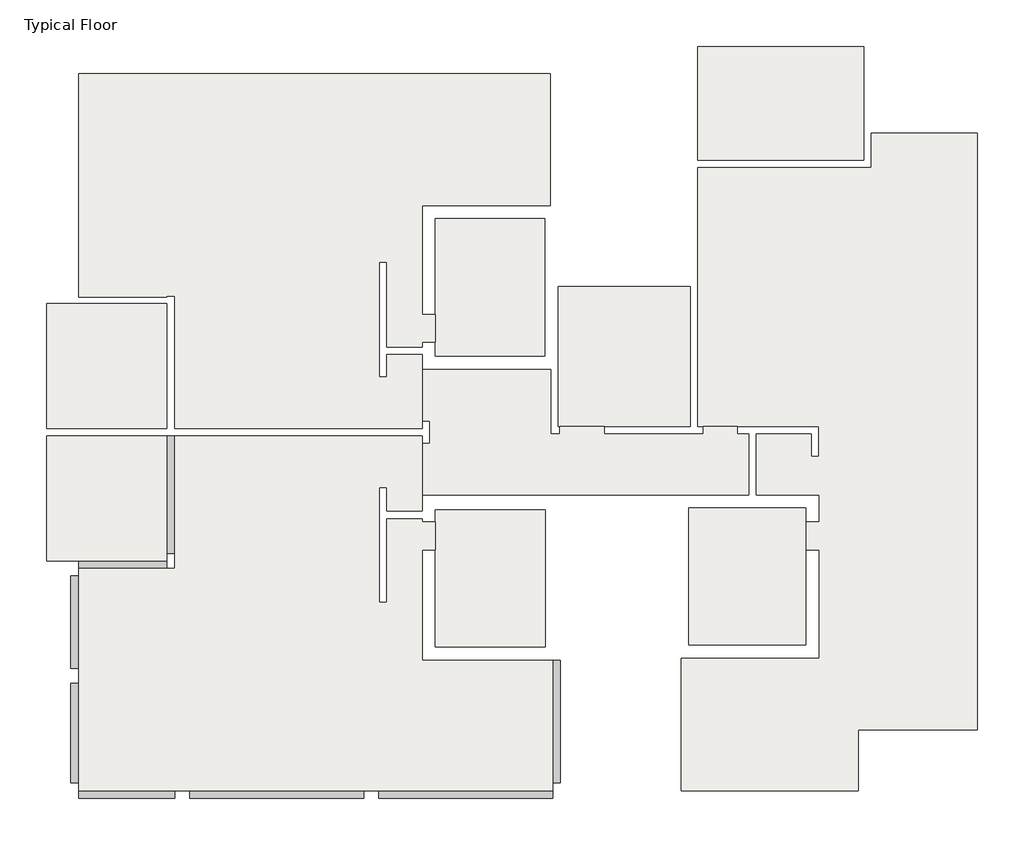
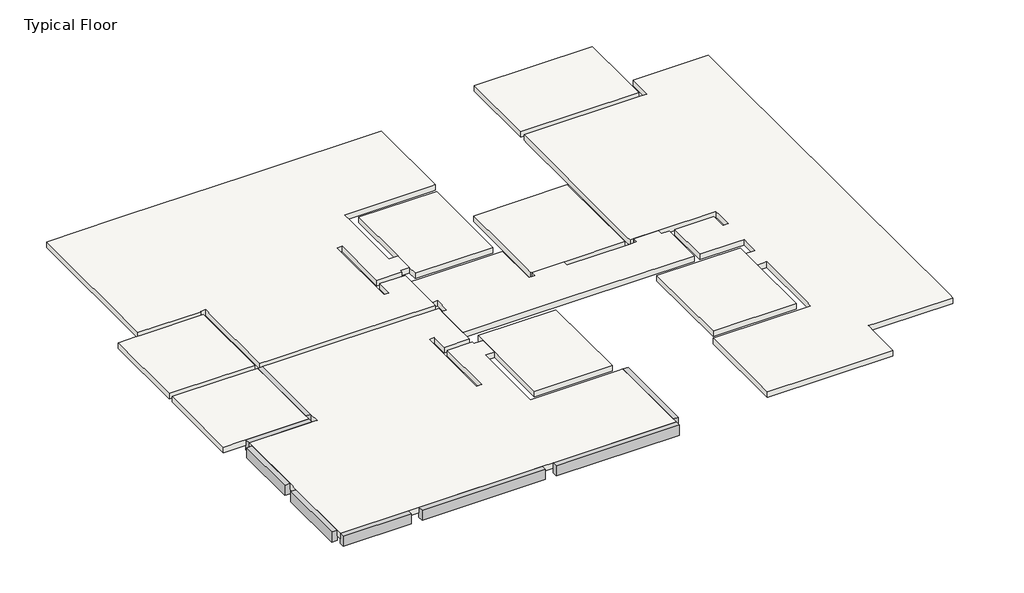
# One storey: 11 slabs, 8 beams.
"""IFC4 building model written with IfcOpenShell, lengths in millimetres."""

from ifc_helpers import new_model, si_unit, frame, origin, place, context, project, spatial, polyline, outline, extrude, faceted_brep, element, save

model = new_model("IFC4")

# Units and contexts
model_context = context("Model", 3, world=origin())
ifc_project = project(units=[si_unit("LENGTHUNIT", "METRE", prefix="MILLI")], contexts=[model_context])

# Site, building, storey
site = spatial("IfcSite", under=ifc_project)
building = spatial("IfcBuilding", under=site)
storey = spatial("IfcBuildingStorey", under=building, Name="Typical Floor", Elevation=3000.0)

# Beams
placement = place(None, origin())
element("IfcBeam", 1, ObjectType="Concrete Rectengular Beam : 20/40", at=placement, inside=storey, context=model_context, shape_type="SweptSolid", body=[
    extrude(outline(polyline([(-8952.4882749, -8486.1299304), (-8952.4882749, -8286.1299304), (-4346.8056177, -8286.1299304), (-4346.8056177, -8486.1299304), (-8952.4882749, -8486.1299304)])), frame((0.0, 0.0, 2600.0), z_axis=(0.0, 0.0, 1.0), x_axis=(1.0, 0.0, 0.0)), (0.0, 0.0, 1.0), 400.0),
])
element("IfcBeam", 2, ObjectType="Concrete Rectengular Beam : 20/40", at=placement, inside=storey, context=model_context, shape_type="Brep", body=[
    faceted_brep([(-11896.6244933, -8286.1299304, 3000.0), (-11896.6244933, -8486.1299304, 3000.0), (-9352.4882749, -8486.1299304, 3000.0), (-9352.4882749, -8286.1299304, 3000.0), (-11896.6244933, -8486.1299304, 2600.0), (-9352.4882749, -8486.1299304, 2600.0), (-11896.6244933, -8286.1299304, 2600.0), (-9352.4882749, -8286.1299304, 2600.0), (-11896.6244933, -8286.1299304, 2780.0)], [[[0, 1, 2, 3]], [[1, 4, 5, 2]], [[4, 6, 7, 5]], [[6, 8, 0, 3, 7]], [[1, 0, 8, 6, 4]], [[3, 2, 5, 7]]]),
])
element("IfcBeam", 3, ObjectType="Concrete Rectengular Beam : 20/40", at=placement, inside=storey, context=model_context, shape_type="SweptSolid", body=[
    extrude(outline(polyline([(-11896.6244933, -8086.1299304), (-12096.6244933, -8086.1299304), (-12096.6244933, -5448.6194614), (-11896.6244933, -5448.6194614), (-11896.6244933, -8086.1299304)])), frame((0.0, 0.0, 2600.0), z_axis=(0.0, 0.0, 1.0), x_axis=(1.0, 0.0, 0.0)), (0.0, 0.0, 1.0), 400.0),
])
element("IfcBeam", 4, ObjectType="Concrete Rectengular Beam : 20/40", at=placement, inside=storey, context=model_context, shape_type="SweptSolid", body=[
    extrude(outline(polyline([(-11896.6244933, -5048.6194614), (-12096.6244933, -5048.6194614), (-12096.6244933, -2598.4826712), (-11896.6244933, -2598.4826712), (-11896.6244933, -5048.6194614)])), frame((0.0, 0.0, 2600.0), z_axis=(0.0, 0.0, 1.0), x_axis=(1.0, 0.0, 0.0)), (0.0, 0.0, 1.0), 400.0),
])
element("IfcBeam", 5, ObjectType="Concrete Rectengular Beam : 20/40", at=placement, inside=storey, context=model_context, shape_type="Brep", body=[
    faceted_brep([(-9554.6843469, -2398.4826712, 3000.0), (-9554.6843469, -2198.4826712, 3000.0), (-11896.6244933, -2198.4826712, 3000.0), (-11896.6244933, -2398.4826712, 3000.0), (-9554.6843469, -2398.4826712, 2600.0), (-9554.6843469, -2398.4826712, 2780.0), (-11896.6244933, -2398.4826712, 2780.0), (-11896.6244933, -2398.4826712, 2600.0), (-9554.6843469, -2198.4826712, 2600.0), (-11896.6244933, -2198.4826712, 2600.0), (-9554.6843469, -2198.4826712, 2780.0)], [[[0, 1, 2, 3]], [[4, 5, 0, 3, 6, 7]], [[8, 4, 7, 9]], [[1, 10, 8, 9, 2]], [[1, 0, 5, 4, 8, 10]], [[3, 2, 9, 7, 6]]]),
])
element("IfcBeam", 6, ObjectType="Concrete Rectengular Beam : 20/40", at=placement, inside=storey, context=model_context, shape_type="Brep", body=[
    faceted_brep([(-9554.6843469, -1998.4826712, 3000.0), (-9354.6843469, -1998.4826712, 3000.0), (-9354.6843469, 1106.8737687, 3000.0), (-9554.6843469, 1106.8737687, 3000.0), (-9554.6843469, -1998.4826712, 2600.0), (-9554.6843469, 1106.8737687, 2780.0), (-9554.6843469, 1106.8737687, 2600.0), (-9354.6843469, -1998.4826712, 2600.0), (-9354.6843469, 1106.8737687, 2600.0), (-9354.6843469, -1998.4826712, 2780.0), (-9354.6843469, 1106.8737687, 2780.0)], [[[0, 1, 2, 3]], [[4, 0, 3, 5, 6]], [[7, 4, 6, 8]], [[1, 9, 7, 8, 10, 2]], [[1, 0, 4, 7, 9]], [[2, 10, 8, 6, 5, 3]]]),
])
element("IfcBeam", 7, ObjectType="Concrete Rectengular Beam : 20/40", at=placement, inside=storey, context=model_context, shape_type="Brep", body=[
    faceted_brep([(-3946.8056177, -8286.1299304, 3000.0), (-3946.8056177, -8486.1299304, 3000.0), (652.6741008, -8486.1299304, 3000.0), (652.6741008, -8286.1299304, 3000.0), (-3946.8056177, -8286.1299304, 2600.0), (652.6741008, -8286.1299304, 2780.0), (652.6741008, -8286.1299304, 2600.0), (-3946.8056177, -8486.1299304, 2600.0), (652.6741008, -8486.1299304, 2600.0)], [[[0, 1, 2, 3]], [[4, 0, 3, 5, 6]], [[7, 4, 6, 8]], [[1, 7, 8, 2]], [[1, 0, 4, 7]], [[3, 2, 8, 6, 5]]]),
])
element("IfcBeam", 8, ObjectType="Concrete Rectengular Beam : 20/40", at=placement, inside=storey, context=model_context, shape_type="Brep", body=[
    faceted_brep([(652.6741008, -8086.1299304, 3000.0), (852.6741008, -8086.1299304, 3000.0), (852.6741008, -4834.488398, 3000.0), (652.6741008, -4834.488398, 3000.0), (652.6741008, -8086.1299304, 2600.0), (652.6741008, -4834.488398, 2780.0), (652.6741008, -4834.488398, 2600.0), (852.6741008, -8086.1299304, 2600.0), (852.6741008, -4834.488398, 2600.0)], [[[0, 1, 2, 3]], [[4, 0, 3, 5, 6]], [[7, 4, 6, 8]], [[1, 7, 8, 2]], [[1, 0, 4, 7]], [[3, 2, 8, 6, 5]]]),
])

# Slabs
element("IfcSlab", 9, ObjectType="22", at=placement, inside=storey, context=model_context, shape_type="SweptSolid", body=[
    extrude(outline(polyline([(447.6741008, 6858.2359353), (447.6741008, 3218.2359353), (-2452.3258992, 3218.2359353), (-2452.3258992, 3588.2359353), (-2457.3258992, 3588.2359353), (-2457.3258992, 4328.2359353), (-2452.3258992, 4328.2359353), (-2452.3258992, 6858.2359353), (447.6741008, 6858.2359353)])), frame((0.0, 0.0, 2780.0), z_axis=(0.0, 0.0, 1.0), x_axis=(1.0, 0.0, 0.0)), (0.0, 0.0, 1.0), 220.0),
])
element("IfcSlab", 10, ObjectType="22", at=placement, inside=storey, context=model_context, shape_type="Brep", body=[
    faceted_brep([(-2802.3258992, 3588.2359353, 2780.0), (-2802.3258992, 3468.2359353, 2780.0), (-3737.2404282, 3468.2359353, 2780.0), (-3737.2404282, 5714.0630881, 2780.0), (-3737.2404282, 5714.3058677, 2780.0), (-3937.2404282, 5714.3058677, 2780.0), (-3937.2404282, 5714.0630881, 2780.0), (-3937.2404282, 2665.7744518, 2780.0), (-3737.2404282, 2665.7744518, 2780.0), (-3737.2404282, 3268.2359353, 2780.0), (-2802.3258992, 3268.2359353, 2780.0), (-2802.3258992, 2868.2359353, 2780.0), (-2800.2213409, 2868.2359353, 2780.0), (-2800.2213409, 1506.8737687, 2780.0), (-2800.2213409, 1306.8737687, 2780.0), (-9354.6843469, 1306.8737687, 2780.0), (-9354.6843469, 4812.2302086, 2780.0), (-9554.6843469, 4812.2302086, 2780.0), (-9554.6843469, 4790.1128337, 2780.0), (-11896.6244933, 4790.1128337, 2780.0), (-11896.6244933, 4812.2302086, 2780.0), (-11896.6244933, 10699.8774677, 2780.0), (592.5229388, 10699.8774677, 2780.0), (592.5229388, 7208.2359353, 2780.0), (447.6741008, 7208.2359353, 2780.0), (-2802.3258992, 7208.2359353, 2780.0), (-2802.3258992, 6858.2359353, 2780.0), (-2802.3258992, 4328.2359353, 2780.0), (-2457.3258992, 4328.2359353, 2780.0), (-2457.3258992, 3588.2359353, 2780.0), (-2802.3258992, 3468.2359353, 3000.0), (-2802.3258992, 3588.2359353, 3000.0), (-2457.3258992, 3588.2359353, 3000.0), (-2457.3258992, 4328.2359353, 3000.0), (-2802.3258992, 4328.2359353, 3000.0), (-2802.3258992, 6858.2359353, 3000.0), (-2802.3258992, 7208.2359353, 3000.0), (447.6741008, 7208.2359353, 3000.0), (592.5229388, 7208.2359353, 3000.0), (592.5229388, 10499.8774677, 3000.0), (592.5229388, 10699.8774677, 3000.0), (-3946.8056177, 10699.8774677, 3000.0), (-4346.8056177, 10699.8774677, 3000.0), (-8952.4882749, 10699.8774677, 3000.0), (-9352.4882749, 10699.8774677, 3000.0), (-11896.6244933, 10699.8774677, 3000.0), (-11896.6244933, 10499.8774677, 3000.0), (-11896.6244933, 7862.3669988, 3000.0), (-11896.6244933, 7462.3669988, 3000.0), (-11896.6244933, 5012.2302086, 3000.0), (-11896.6244933, 4790.1128337, 3000.0), (-9554.6843469, 4790.1128337, 3000.0), (-9554.6843469, 4812.2302086, 3000.0), (-9354.6843469, 4812.2302086, 3000.0), (-9354.6843469, 4412.2302086, 3000.0), (-9354.6843469, 1306.8737687, 3000.0), (-8954.6843469, 1306.8737687, 3000.0), (-6260.2213409, 1306.8737687, 3000.0), (-5860.2213409, 1306.8737687, 3000.0), (-2800.2213409, 1306.8737687, 3000.0), (-2800.2213409, 1506.8737687, 3000.0), (-2800.2213409, 2868.2359353, 3000.0), (-2802.3258992, 2868.2359353, 3000.0), (-2802.3258992, 3268.2359353, 3000.0), (-3737.2404282, 3268.2359353, 3000.0), (-3737.2404282, 2665.7744518, 3000.0), (-3937.2404282, 2665.7744518, 3000.0), (-3937.2404282, 5714.0630881, 3000.0), (-3937.2404282, 5714.3058677, 3000.0), (-3737.2404282, 5714.3058677, 3000.0), (-3737.2404282, 5714.0630881, 3000.0), (-3737.2404282, 3468.2359353, 3000.0)], [[[0, 1, 2, 3, 4, 5, 6, 7, 8, 9, 10, 11, 12, 13, 14, 15, 16, 17, 18, 19, 20, 21, 22, 23, 24, 25, 26, 27, 28, 29]], [[30, 31, 32, 33, 34, 35, 36, 37, 38, 39, 40, 41, 42, 43, 44, 45, 46, 47, 48, 49, 50, 51, 52, 53, 54, 55, 56, 57, 58, 59, 60, 61, 62, 63, 64, 65, 66, 67, 68, 69, 70, 71]], [[27, 34, 33, 28]], [[31, 0, 29, 32]], [[1, 0, 31, 30]], [[2, 1, 30, 71]], [[2, 71, 70, 69, 4, 3]], [[5, 4, 69, 68]], [[5, 68, 67, 66, 7, 6]], [[8, 7, 66, 65]], [[9, 8, 65, 64]], [[9, 64, 63, 10]], [[59, 14, 13, 12, 61, 60]], [[15, 14, 59, 58, 57, 56, 55]], [[15, 55, 54, 53, 16]], [[50, 19, 18, 51]], [[21, 20, 19, 50, 49, 48, 47, 46, 45]], [[22, 21, 45, 44, 43, 42, 41, 40]], [[23, 22, 40, 39, 38]], [[23, 38, 37, 36, 25, 24]], [[25, 36, 35, 34, 27, 26]], [[17, 52, 51, 18]], [[52, 17, 16, 53]], [[62, 11, 10, 63]], [[11, 62, 61, 12]], [[29, 28, 33, 32]]]),
])
element("IfcSlab", 11, ObjectType="22", at=placement, inside=storey, context=model_context, shape_type="Brep", body=[
    faceted_brep([(-12743.1090323, 4612.2302086, 2780.0), (-9554.6843469, 4612.2302086, 2780.0), (-9554.6843469, 1306.8737687, 2780.0), (-12743.1090323, 1306.8737687, 2780.0), (-9554.6843469, 4612.2302086, 3000.0), (-11896.6244933, 4612.2302086, 3000.0), (-12096.6244933, 4612.2302086, 3000.0), (-12743.1090323, 4612.2302086, 3000.0), (-12743.1090323, 1306.8737687, 3000.0), (-12343.1090323, 1306.8737687, 3000.0), (-9954.6843469, 1306.8737687, 3000.0), (-9554.6843469, 1306.8737687, 3000.0), (-9554.6843469, 4412.2302086, 3000.0)], [[[0, 1, 2, 3]], [[4, 5, 6, 7, 8, 9, 10, 11, 12]], [[1, 0, 7, 6, 5, 4]], [[2, 1, 4, 12, 11]], [[3, 2, 11, 10, 9, 8]], [[0, 3, 8, 7]]]),
])
element("IfcSlab", 12, ObjectType="22", at=placement, inside=storey, context=model_context, shape_type="Brep", body=[
    faceted_brep([(452.6741008, -4484.488398, 2780.0), (-2452.3258992, -4484.488398, 2780.0), (-2452.3258992, -1914.488398, 2780.0), (-2452.3258992, -1174.488398, 2780.0), (-2452.3258992, -854.488398, 2780.0), (452.6741008, -854.488398, 2780.0), (452.6741008, -4484.488398, 3000.0), (452.6741008, -854.488398, 3000.0), (-2452.3258992, -854.488398, 3000.0), (-2452.3258992, -1174.488398, 3000.0), (-2452.3258992, -1914.488398, 3000.0), (-2452.3258992, -4484.488398, 3000.0)], [[[0, 1, 2, 3, 4, 5]], [[6, 7, 8, 9, 10, 11]], [[0, 5, 7, 6]], [[5, 4, 8, 7]], [[4, 3, 2, 1, 11, 10, 9, 8]], [[1, 0, 6, 11]]]),
])
element("IfcSlab", 13, ObjectType="22", at=placement, inside=storey, context=model_context, shape_type="Brep", body=[
    faceted_brep([(-2452.3258992, -1914.488398, 2780.0), (-2802.3258992, -1914.488398, 2780.0), (-2802.3258992, -4484.488398, 2780.0), (-2802.3258992, -4834.488398, 2780.0), (452.6741008, -4834.488398, 2780.0), (652.6741008, -4834.488398, 2780.0), (652.6741008, -8286.1299304, 2780.0), (-11896.6244933, -8286.1299304, 2780.0), (-11896.6244933, -2398.4826712, 2780.0), (-9554.6843469, -2398.4826712, 2780.0), (-9354.6843469, -2398.4826712, 2780.0), (-9354.6843469, -1998.4826712, 2780.0), (-9354.6843469, 1106.8737687, 2780.0), (-2800.2213409, 1106.8737687, 2780.0), (-2800.2213409, 906.8737687, 2780.0), (-2800.2213409, -454.488398, 2780.0), (-2802.3258992, -454.488398, 2780.0), (-2802.3258992, -884.488398, 2780.0), (-3737.2404282, -884.488398, 2780.0), (-3737.2404282, -252.0269144, 2780.0), (-3937.2404282, -252.0269144, 2780.0), (-3937.2404282, -3300.3155508, 2780.0), (-3937.2404282, -3300.5583304, 2780.0), (-3737.2404282, -3300.5583304, 2780.0), (-3737.2404282, -3300.3155508, 2780.0), (-3737.2404282, -1084.488398, 2780.0), (-2802.3258992, -1084.488398, 2780.0), (-2802.3258992, -1174.488398, 2780.0), (-2452.3258992, -1174.488398, 2780.0), (-2802.3258992, -1914.488398, 3000.0), (-2452.3258992, -1914.488398, 3000.0), (-2452.3258992, -1174.488398, 3000.0), (-2802.3258992, -1174.488398, 3000.0), (-2802.3258992, -1084.488398, 3000.0), (-3737.2404282, -1084.488398, 3000.0), (-3737.2404282, -3300.3155508, 3000.0), (-3737.2404282, -3300.5583304, 3000.0), (-3937.2404282, -3300.5583304, 3000.0), (-3937.2404282, -3300.3155508, 3000.0), (-3937.2404282, -252.0269144, 3000.0), (-3737.2404282, -252.0269144, 3000.0), (-3737.2404282, -884.488398, 3000.0), (-2802.3258992, -884.488398, 3000.0), (-2802.3258992, -454.488398, 3000.0), (-2800.2213409, -454.488398, 3000.0), (-2800.2213409, 906.8737687, 3000.0), (-2800.2213409, 1106.8737687, 3000.0), (-5860.2213409, 1106.8737687, 3000.0), (-6260.2213409, 1106.8737687, 3000.0), (-8954.6843469, 1106.8737687, 3000.0), (-9354.6843469, 1106.8737687, 3000.0), (-9354.6843469, -1998.4826712, 3000.0), (-9354.6843469, -2398.4826712, 3000.0), (-9554.6843469, -2398.4826712, 3000.0), (-11896.6244933, -2398.4826712, 3000.0), (-11896.6244933, -2598.4826712, 3000.0), (-11896.6244933, -5048.6194614, 3000.0), (-11896.6244933, -5448.6194614, 3000.0), (-11896.6244933, -8086.1299304, 3000.0), (-11896.6244933, -8286.1299304, 3000.0), (-9352.4882749, -8286.1299304, 3000.0), (-8952.4882749, -8286.1299304, 3000.0), (-4346.8056177, -8286.1299304, 3000.0), (-3946.8056177, -8286.1299304, 3000.0), (652.6741008, -8286.1299304, 3000.0), (652.6741008, -8086.1299304, 3000.0), (652.6741008, -4834.488398, 3000.0), (452.6741008, -4834.488398, 3000.0), (-2802.3258992, -4834.488398, 3000.0), (-2802.3258992, -4484.488398, 3000.0)], [[[0, 1, 2, 3, 4, 5, 6, 7, 8, 9, 10, 11, 12, 13, 14, 15, 16, 17, 18, 19, 20, 21, 22, 23, 24, 25, 26, 27, 28]], [[29, 30, 31, 32, 33, 34, 35, 36, 37, 38, 39, 40, 41, 42, 43, 44, 45, 46, 47, 48, 49, 50, 51, 52, 53, 54, 55, 56, 57, 58, 59, 60, 61, 62, 63, 64, 65, 66, 67, 68, 69]], [[1, 0, 30, 29]], [[0, 28, 31, 30]], [[28, 27, 32, 31]], [[27, 26, 33, 32]], [[26, 25, 34, 33]], [[23, 36, 35, 34, 25, 24]], [[23, 22, 37, 36]], [[20, 39, 38, 37, 22, 21]], [[20, 19, 40, 39]], [[19, 18, 41, 40]], [[41, 18, 17, 42]], [[13, 46, 45, 44, 15, 14]], [[13, 12, 50, 49, 48, 47, 46]], [[10, 52, 51, 50, 12, 11]], [[8, 54, 53, 52, 10, 9]], [[8, 7, 59, 58, 57, 56, 55, 54]], [[7, 6, 64, 63, 62, 61, 60, 59]], [[6, 5, 66, 65, 64]], [[3, 68, 67, 66, 5, 4]], [[68, 3, 2, 1, 29, 69]], [[16, 43, 42, 17]], [[43, 16, 15, 44]]]),
])
element("IfcSlab", 14, ObjectType="22", at=placement, inside=storey, context=model_context, shape_type="Brep", body=[
    faceted_brep([(-9554.6843469, -2198.4826712, 2780.0), (-12743.1090323, -2198.4826712, 2780.0), (-12743.1090323, 1106.8737687, 2780.0), (-9554.6843469, 1106.8737687, 2780.0), (-12743.1090323, -2198.4826712, 3000.0), (-12096.6244933, -2198.4826712, 3000.0), (-11896.6244933, -2198.4826712, 3000.0), (-9554.6843469, -2198.4826712, 3000.0), (-9554.6843469, -1998.4826712, 3000.0), (-9554.6843469, 1106.8737687, 3000.0), (-9954.6843469, 1106.8737687, 3000.0), (-12343.1090323, 1106.8737687, 3000.0), (-12743.1090323, 1106.8737687, 3000.0)], [[[0, 1, 2, 3]], [[4, 5, 6, 7, 8, 9, 10, 11, 12]], [[1, 0, 7, 6, 5, 4]], [[0, 3, 9, 8, 7]], [[3, 2, 12, 11, 10, 9]], [[2, 1, 4, 12]]]),
])
element("IfcSlab", 15, ObjectType="22", at=placement, inside=storey, context=model_context, shape_type="Brep", body=[
    faceted_brep([(7355.8942254, -4432.6671723, 2780.0), (4252.6741008, -4432.6671723, 2780.0), (4252.6741008, -804.488398, 2780.0), (7355.8942254, -804.488398, 2780.0), (7355.8942254, -1174.488398, 2780.0), (7355.8942254, -1914.488398, 2780.0), (4252.6741008, -4432.6671723, 3000.0), (7355.8942254, -4432.6671723, 3000.0), (7355.8942254, -1914.488398, 3000.0), (7355.8942254, -1174.488398, 3000.0), (7355.8942254, -804.488398, 3000.0), (4252.6741008, -804.488398, 3000.0)], [[[0, 1, 2, 3, 4, 5]], [[6, 7, 8, 9, 10, 11]], [[1, 6, 11, 2]], [[7, 0, 5, 4, 3, 10, 9, 8]], [[1, 0, 7, 6]], [[3, 2, 11, 10]]]),
])
element("IfcSlab", 16, ObjectType="22", at=placement, inside=storey, context=model_context, shape_type="Brep", body=[
    faceted_brep([(4052.6741008, -8286.1299304, 2780.0), (4052.6741008, -4782.6671723, 2780.0), (4252.6741008, -4782.6671723, 2780.0), (7705.8942254, -4782.6671723, 2780.0), (7705.8942254, -4432.6671723, 2780.0), (7705.8942254, -1914.488398, 2780.0), (7355.8942254, -1914.488398, 2780.0), (7355.8942254, -1174.488398, 2780.0), (7705.8942254, -1174.488398, 2780.0), (7705.8942254, -454.488398, 2780.0), (7355.8942254, -454.488398, 2780.0), (6043.815032, -454.488398, 2780.0), (6043.815032, 1157.9050688, 2780.0), (7503.815032, 1157.9050688, 2780.0), (7503.815032, 565.511602, 2780.0), (7703.815032, 565.511602, 2780.0), (7703.815032, 1157.9050688, 2780.0), (7703.815032, 1357.9050688, 2780.0), (5543.815032, 1357.9050688, 2780.0), (4640.5760436, 1357.9050688, 2780.0), (4497.0462143, 1357.9050688, 2780.0), (4497.0462143, 1557.9050688, 2780.0), (4497.0462143, 4964.8955051, 2780.0), (4497.0462143, 5364.8955051, 2780.0), (4497.0462143, 8011.9737794, 2780.0), (4497.0462143, 8211.9737794, 2780.0), (8895.1583714, 8211.9737794, 2780.0), (9095.1583714, 8211.9737794, 2780.0), (9095.1583714, 8411.9737794, 2780.0), (9095.1583714, 9122.6036006, 2780.0), (11900.0250654, 9122.6036006, 2780.0), (11900.0250654, -6681.7453909, 2780.0), (9346.3765637, -6681.7453909, 2780.0), (8946.3765637, -6681.7453909, 2780.0), (8746.3765637, -6681.7453909, 2780.0), (8746.3765637, -7081.7453909, 2780.0), (8746.3765637, -8086.1299304, 2780.0), (8746.3765637, -8286.1299304, 2780.0), (4052.6741008, -4782.6671723, 3000.0), (4052.6741008, -8086.1299304, 3000.0), (4052.6741008, -8286.1299304, 3000.0), (5752.5819696, -8286.1299304, 3000.0), (6152.5819696, -8286.1299304, 3000.0), (8746.3765637, -8286.1299304, 3000.0), (8746.3765637, -8086.1299304, 3000.0), (8746.3765637, -7081.7453909, 3000.0), (8746.3765637, -6681.7453909, 3000.0), (8946.3765637, -6681.7453909, 3000.0), (9346.3765637, -6681.7453909, 3000.0), (11900.0250654, -6681.7453909, 3000.0), (11900.0250654, -6481.7453909, 3000.0), (11900.0250654, -3292.2632704, 3000.0), (11900.0250654, -2892.2632704, 3000.0), (11900.0250654, -1042.5387376, 3000.0), (11900.0250654, -642.5387376, 3000.0), (11900.0250654, 2306.6846493, 3000.0), (11900.0250654, 2706.6846493, 3000.0), (11900.0250654, 5508.9593048, 3000.0), (11900.0250654, 5908.9593048, 3000.0), (11900.0250654, 8922.6036006, 3000.0), (11900.0250654, 9122.6036006, 3000.0), (9095.1583714, 9122.6036006, 3000.0), (9095.1583714, 8411.9737794, 3000.0), (9095.1583714, 8211.9737794, 3000.0), (8895.1583714, 8211.9737794, 3000.0), (4497.0462143, 8211.9737794, 3000.0), (4497.0462143, 8011.9737794, 3000.0), (4497.0462143, 5364.8955051, 3000.0), (4497.0462143, 4964.8955051, 3000.0), (4497.0462143, 1557.9050688, 3000.0), (4497.0462143, 1357.9050688, 3000.0), (4640.5760436, 1357.9050688, 3000.0), (5543.815032, 1357.9050688, 3000.0), (7703.815032, 1357.9050688, 3000.0), (7703.815032, 1157.9050688, 3000.0), (7703.815032, 565.511602, 3000.0), (7503.815032, 565.511602, 3000.0), (7503.815032, 1157.9050688, 3000.0), (6043.815032, 1157.9050688, 3000.0), (6043.815032, -454.488398, 3000.0), (7355.8942254, -454.488398, 3000.0), (7705.8942254, -454.488398, 3000.0), (7705.8942254, -1174.488398, 3000.0), (7355.8942254, -1174.488398, 3000.0), (7355.8942254, -1914.488398, 3000.0), (7705.8942254, -1914.488398, 3000.0), (7705.8942254, -4432.6671723, 3000.0), (7705.8942254, -4782.6671723, 3000.0), (4252.6741008, -4782.6671723, 3000.0)], [[[0, 1, 2, 3, 4, 5, 6, 7, 8, 9, 10, 11, 12, 13, 14, 15, 16, 17, 18, 19, 20, 21, 22, 23, 24, 25, 26, 27, 28, 29, 30, 31, 32, 33, 34, 35, 36, 37]], [[38, 39, 40, 41, 42, 43, 44, 45, 46, 47, 48, 49, 50, 51, 52, 53, 54, 55, 56, 57, 58, 59, 60, 61, 62, 63, 64, 65, 66, 67, 68, 69, 70, 71, 72, 73, 74, 75, 76, 77, 78, 79, 80, 81, 82, 83, 84, 85, 86, 87, 88]], [[1, 0, 40, 39, 38]], [[1, 38, 88, 87, 3, 2]], [[3, 87, 86, 85, 5, 4]], [[6, 5, 85, 84]], [[7, 6, 84, 83]], [[8, 7, 83, 82]], [[9, 8, 82, 81]], [[9, 81, 80, 79, 11, 10]], [[12, 11, 79, 78]], [[13, 12, 78, 77]], [[14, 13, 77, 76]], [[15, 14, 76, 75]], [[15, 75, 74, 73, 17, 16]], [[18, 17, 73, 72]], [[19, 18, 72, 71]], [[20, 19, 71, 70]], [[20, 70, 69, 68, 67, 66, 65, 25, 24, 23, 22, 21]], [[25, 65, 64, 63, 27, 26]], [[27, 63, 62, 61, 29, 28]], [[30, 29, 61, 60]], [[31, 30, 60, 59, 58, 57, 56, 55, 54, 53, 52, 51, 50, 49]], [[31, 49, 48, 47, 46, 34, 33, 32]], [[34, 46, 45, 44, 43, 37, 36, 35]], [[0, 37, 43, 42, 41, 40]]]),
])
element("IfcSlab", 17, ObjectType="22", at=placement, inside=storey, context=model_context, shape_type="Brep", body=[
    faceted_brep([(5543.815032, 1157.9050688, 2780.0), (5843.815032, 1157.9050688, 2780.0), (5843.815032, -454.488398, 2780.0), (-2800.2213409, -454.488398, 2780.0), (-2800.2213409, 906.8737687, 2780.0), (-2600.2213409, 906.8737687, 2780.0), (-2600.2213409, 1506.8737687, 2780.0), (-2800.2213409, 1506.8737687, 2780.0), (-2800.2213409, 2868.2359353, 2780.0), (597.6741008, 2868.2359353, 2780.0), (597.6741008, 1357.9050688, 2780.0), (597.6741008, 1157.9050688, 2780.0), (842.9874073, 1157.9050688, 2780.0), (842.9874073, 1357.9050688, 2780.0), (2014.3086194, 1357.9050688, 2780.0), (2014.3086194, 1157.9050688, 2780.0), (4297.0462143, 1157.9050688, 2780.0), (4495.5760436, 1157.9050688, 2780.0), (4497.0462143, 1157.9050688, 2780.0), (4640.5760436, 1157.9050688, 2780.0), (4640.5760436, 1357.9050688, 2780.0), (5543.815032, 1357.9050688, 2780.0), (5843.815032, 1157.9050688, 3000.0), (5543.815032, 1157.9050688, 3000.0), (5543.815032, 1357.9050688, 3000.0), (4640.5760436, 1357.9050688, 3000.0), (4640.5760436, 1157.9050688, 3000.0), (4497.0462143, 1157.9050688, 3000.0), (4495.5760436, 1157.9050688, 3000.0), (4297.0462143, 1157.9050688, 3000.0), (2014.3086194, 1157.9050688, 3000.0), (2014.3086194, 1357.9050688, 3000.0), (842.9874073, 1357.9050688, 3000.0), (842.9874073, 1157.9050688, 3000.0), (597.6741008, 1157.9050688, 3000.0), (597.6741008, 1357.9050688, 3000.0), (597.6741008, 2868.2359353, 3000.0), (-2452.3258992, 2868.2359353, 3000.0), (-2800.2213409, 2868.2359353, 3000.0), (-2800.2213409, 1506.8737687, 3000.0), (-2600.2213409, 1506.8737687, 3000.0), (-2600.2213409, 906.8737687, 3000.0), (-2800.2213409, 906.8737687, 3000.0), (-2800.2213409, -454.488398, 3000.0), (-2452.3258992, -454.488398, 3000.0), (852.6741008, -454.488398, 3000.0), (3852.6741008, -454.488398, 3000.0), (5843.815032, -454.488398, 3000.0)], [[[0, 1, 2, 3, 4, 5, 6, 7, 8, 9, 10, 11, 12, 13, 14, 15, 16, 17, 18, 19, 20, 21]], [[22, 23, 24, 25, 26, 27, 28, 29, 30, 31, 32, 33, 34, 35, 36, 37, 38, 39, 40, 41, 42, 43, 44, 45, 46, 47]], [[1, 0, 23, 22]], [[2, 1, 22, 47]], [[2, 47, 46, 45, 44, 43, 3]], [[41, 5, 4, 42]], [[39, 7, 6, 40]], [[8, 7, 39, 38]], [[9, 8, 38, 37, 36]], [[9, 36, 35, 34, 11, 10]], [[12, 11, 34, 33]], [[13, 12, 33, 32]], [[14, 13, 32, 31]], [[15, 14, 31, 30]], [[15, 30, 29, 28, 27, 26, 19, 18, 17, 16]], [[20, 19, 26, 25]], [[21, 20, 25, 24]], [[0, 21, 24, 23]], [[5, 41, 40, 6]], [[4, 3, 43, 42]]]),
])
element("IfcSlab", 18, ObjectType="22", at=placement, inside=storey, context=model_context, shape_type="Brep", body=[
    faceted_brep([(4497.0462143, 11422.6036006, 2780.0), (8895.1583714, 11422.6036006, 2780.0), (8895.1583714, 8411.9737794, 2780.0), (4497.0462143, 8411.9737794, 2780.0), (8895.1583714, 11422.6036006, 3000.0), (4497.0462143, 11422.6036006, 3000.0), (4497.0462143, 8411.9737794, 3000.0), (8895.1583714, 8411.9737794, 3000.0), (8895.1583714, 9122.6036006, 3000.0), (8895.1583714, 9322.6036006, 3000.0)], [[[0, 1, 2, 3]], [[4, 5, 6, 7, 8, 9]], [[1, 0, 5, 4]], [[2, 1, 4, 9, 8, 7]], [[3, 2, 7, 6]], [[0, 3, 6, 5]]]),
])
element("IfcSlab", 19, ObjectType="22", at=placement, inside=storey, context=model_context, shape_type="Brep", body=[
    faceted_brep([(4297.0462143, 5064.8955051, 2780.0), (4297.0462143, 1357.9050688, 2780.0), (2014.3086194, 1357.9050688, 2780.0), (842.9874073, 1357.9050688, 2780.0), (797.6741008, 1357.9050688, 2780.0), (797.6741008, 5064.8955051, 2780.0), (4297.0462143, 1357.9050688, 3000.0), (4297.0462143, 1557.9050688, 3000.0), (4297.0462143, 4964.8955051, 3000.0), (4297.0462143, 5064.8955051, 3000.0), (797.6741008, 5064.8955051, 3000.0), (797.6741008, 3218.2359353, 3000.0), (797.6741008, 2868.2359353, 3000.0), (797.6741008, 1357.9050688, 3000.0), (842.9874073, 1357.9050688, 3000.0), (2014.3086194, 1357.9050688, 3000.0)], [[[0, 1, 2, 3, 4, 5]], [[6, 7, 8, 9, 10, 11, 12, 13, 14, 15]], [[1, 0, 9, 8, 7, 6]], [[1, 6, 15, 14, 13, 4, 3, 2]], [[9, 0, 5, 10]], [[10, 5, 4, 13, 12, 11]]]),
])

save(model, "model.ifc")

# Revit data of these elements
# Type "Concrete Rectengular Beam : 20/40"
#   Keynote = "09000"
#   Length [instance default] = 152.4 cm
#   b = 20 cm
#   h = 40 cm
#   Structural Material [instance default] = Concrete
#   Assembly Code = ""
# Type "22"
#   Function = 0
#   Layers, outside or top first: 22 cm "Concrete" (function 1)
# Element 1 (IfcBeam, "Concrete Rectengular Beam : 20/40")
#   Comments = ""
#   Mark = "B12"
#   SOFiSTiK_AMG_Comments = ""
#   SOFiSTiK_AMG_Scheduled = yes
#   SOFiSTiK_AMG_Adjusted = yes
#   Structural Material = Concrete
#   Phase Created = New Construction
#   Materials on its faces: "Concrete"
# Element 2 (IfcBeam, "Concrete Rectengular Beam : 20/40")
#   Comments = ""
#   Mark = "B13"
#   SOFiSTiK_AMG_Comments = ""
#   SOFiSTiK_AMG_Scheduled = yes
#   SOFiSTiK_AMG_Adjusted = yes
#   Structural Material = Concrete
#   Phase Created = New Construction
#   Materials on its faces: "Concrete"
# Element 3 (IfcBeam, "Concrete Rectengular Beam : 20/40")
#   Comments = ""
#   Mark = "B14"
#   SOFiSTiK_AMG_Comments = ""
#   SOFiSTiK_AMG_Scheduled = yes
#   SOFiSTiK_AMG_Adjusted = yes
#   Structural Material = Concrete
#   Phase Created = New Construction
#   Materials on its faces: "Concrete"
# Element 4 (IfcBeam, "Concrete Rectengular Beam : 20/40")
#   Comments = ""
#   Mark = "B15"
#   SOFiSTiK_AMG_Comments = ""
#   SOFiSTiK_AMG_Scheduled = yes
#   SOFiSTiK_AMG_Adjusted = yes
#   Structural Material = Concrete
#   Phase Created = New Construction
#   Materials on its faces: "Concrete"
# Element 5 (IfcBeam, "Concrete Rectengular Beam : 20/40")
#   Comments = ""
#   Mark = "B16"
#   SOFiSTiK_AMG_Comments = ""
#   SOFiSTiK_AMG_Scheduled = yes
#   SOFiSTiK_AMG_Adjusted = yes
#   Structural Material = Concrete
#   Phase Created = New Construction
#   Materials on its faces: "Concrete"
# Element 6 (IfcBeam, "Concrete Rectengular Beam : 20/40")
#   Comments = ""
#   Mark = "B17"
#   SOFiSTiK_AMG_Comments = ""
#   SOFiSTiK_AMG_Scheduled = yes
#   SOFiSTiK_AMG_Adjusted = yes
#   Structural Material = Concrete
#   Phase Created = New Construction
#   Materials on its faces: "Concrete"
# Element 7 (IfcBeam, "Concrete Rectengular Beam : 20/40")
#   Comments = ""
#   Mark = "B18"
#   SOFiSTiK_AMG_Comments = ""
#   SOFiSTiK_AMG_Scheduled = yes
#   SOFiSTiK_AMG_Adjusted = yes
#   Structural Material = Concrete
#   Phase Created = New Construction
#   Materials on its faces: "Concrete"
# Element 8 (IfcBeam, "Concrete Rectengular Beam : 20/40")
#   Comments = ""
#   Mark = "B19"
#   SOFiSTiK_AMG_Comments = ""
#   SOFiSTiK_AMG_Scheduled = yes
#   SOFiSTiK_AMG_Adjusted = yes
#   Structural Material = Concrete
#   Phase Created = New Construction
#   Materials on its faces: "Concrete"
# Element 9 (IfcSlab, "22")
#   Mark = "S1"
#   SOFiSTiK_AMG_Comments = ""
#   Height Offset From Level = 0 cm
#   built-in parameter 1001954 = 1
#   SOFiSTiK_AMG_Scheduled = yes
#   SOFiSTiK_AMG_Adjusted = yes
#   Phase Created = New Construction
#   Materials on its faces: "Concrete"
# Element 10 (IfcSlab, "22")
#   Mark = "S2"
#   SOFiSTiK_AMG_Comments = ""
#   built-in parameter 1001955 = 3.14159 (stored number, unit not read)
#   Height Offset From Level = 0 cm
#   built-in parameter 1001954 = 1
#   SOFiSTiK_AMG_Scheduled = yes
#   SOFiSTiK_AMG_Adjusted = yes
#   Phase Created = New Construction
#   Materials on its faces: "Concrete"
# Element 11 (IfcSlab, "22")
#   Mark = "S3"
#   SOFiSTiK_AMG_Comments = ""
#   built-in parameter 1001955 = 3.14159 (stored number, unit not read)
#   Height Offset From Level = 0 cm
#   built-in parameter 1001954 = 1
#   SOFiSTiK_AMG_Scheduled = yes
#   SOFiSTiK_AMG_Adjusted = yes
#   Phase Created = New Construction
#   Materials on its faces: "Concrete"
# Element 12 (IfcSlab, "22")
#   Mark = "S4"
#   SOFiSTiK_AMG_Comments = ""
#   Height Offset From Level = 0 cm
#   built-in parameter 1001954 = 1
#   SOFiSTiK_AMG_Scheduled = yes
#   SOFiSTiK_AMG_Adjusted = yes
#   Phase Created = New Construction
#   Materials on its faces: "Concrete"
# Element 13 (IfcSlab, "22")
#   Mark = "S5"
#   SOFiSTiK_AMG_Comments = ""
#   built-in parameter 1001955 = 3.14159 (stored number, unit not read)
#   Height Offset From Level = 0 cm
#   built-in parameter 1001954 = 1
#   SOFiSTiK_AMG_Scheduled = yes
#   SOFiSTiK_AMG_Adjusted = yes
#   Phase Created = New Construction
#   Materials on its faces: "Concrete"
# Element 14 (IfcSlab, "22")
#   Mark = "S6"
#   SOFiSTiK_AMG_Comments = ""
#   built-in parameter 1001955 = 3.14159 (stored number, unit not read)
#   Height Offset From Level = 0 cm
#   built-in parameter 1001954 = 1
#   SOFiSTiK_AMG_Scheduled = yes
#   SOFiSTiK_AMG_Adjusted = yes
#   Phase Created = New Construction
#   Materials on its faces: "Concrete"
# Element 15 (IfcSlab, "22")
#   Mark = "S7"
#   SOFiSTiK_AMG_Comments = ""
#   built-in parameter 1001955 = 3.14159 (stored number, unit not read)
#   Height Offset From Level = 0 cm
#   built-in parameter 1001954 = 1
#   SOFiSTiK_AMG_Scheduled = yes
#   SOFiSTiK_AMG_Adjusted = yes
#   Phase Created = New Construction
#   Materials on its faces: "Concrete"
# Element 16 (IfcSlab, "22")
#   Mark = "S8"
#   SOFiSTiK_AMG_Comments = ""
#   built-in parameter 1001955 = -1.5708 (stored number, unit not read)
#   Height Offset From Level = 0 cm
#   built-in parameter 1001954 = 1
#   SOFiSTiK_AMG_Scheduled = yes
#   SOFiSTiK_AMG_Adjusted = yes
#   Phase Created = New Construction
#   Materials on its faces: "Concrete"
# Element 17 (IfcSlab, "22")
#   Mark = "S9"
#   SOFiSTiK_AMG_Comments = ""
#   built-in parameter 1001955 = -1.5708 (stored number, unit not read)
#   Height Offset From Level = 0 cm
#   built-in parameter 1001954 = 1
#   SOFiSTiK_AMG_Scheduled = yes
#   SOFiSTiK_AMG_Adjusted = no
#   Phase Created = New Construction
#   Materials on its faces: "Concrete"
# Element 18 (IfcSlab, "22")
#   Mark = "S10"
#   SOFiSTiK_AMG_Comments = ""
#   built-in parameter 1001955 = 3.14159 (stored number, unit not read)
#   Height Offset From Level = 0 cm
#   built-in parameter 1001954 = 1
#   SOFiSTiK_AMG_Scheduled = yes
#   SOFiSTiK_AMG_Adjusted = yes
#   Phase Created = New Construction
#   Materials on its faces: "Concrete"
# Element 19 (IfcSlab, "22")
#   Mark = "S11"
#   SOFiSTiK_AMG_Comments = ""
#   Height Offset From Level = 0 cm
#   built-in parameter 1001954 = 1
#   SOFiSTiK_AMG_Scheduled = yes
#   SOFiSTiK_AMG_Adjusted = yes
#   Phase Created = New Construction
#   Materials on its faces: "Concrete"
# Materials
#   "Concrete": class "Concrete", colour RGB 192 192 192, transparency 0, Keynote = "01000", Description = "Cast-in-place concrete", Cost = 0
